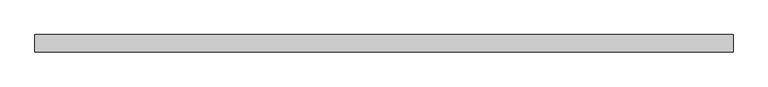
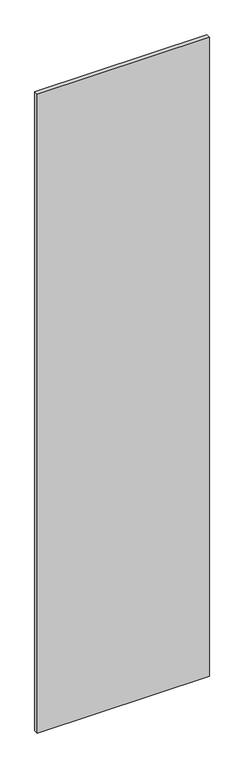
"""IFC4 building model written with IfcOpenShell, lengths in millimetres: plate geometry, 系统嵌板 : 玻璃."""

import ifcopenshell
import ifcopenshell.guid

model = None  # the IFC model being written
_history = None  # IfcOwnerHistory: only IFC2X3 demands one
_inside = {}  # id of a spatial element -> (the spatial element, [elements in it])
_under = {}  # id of a project, library or spatial element -> (it, [spatial elements below it])
_declared = {}  # id of a project -> (the project, [libraries it declares])
_typed = {}  # id of a type object -> (the type object, [elements of that type])
_made_of = {}  # id of a material, layer set ... -> (it, [elements and type objects made of it])


def new_model(schema):
    """Start an empty IFC model of exactly this schema.

    Asked for "IFC4X3", IfcOpenShell would pick the latest addendum, in which some entities
    have other attributes; the version numbers below select the first issue.
    IFC2X3 requires an IfcOwnerHistory on every rooted entity: one is made here for all.
    """
    global model, _history
    if schema == "IFC4X3":
        model = ifcopenshell.file(schema_version=(4, 3, 0, 0))
    else:
        model = ifcopenshell.file(schema=schema)
    _inside.clear()
    _under.clear()
    _declared.clear()
    _typed.clear()
    _made_of.clear()
    _history = None
    if model.schema == "IFC2X3":
        org = make("IfcOrganization", Name="unknown")
        user = make(
            "IfcPersonAndOrganization",
            ThePerson=make("IfcPerson", FamilyName="unknown"),
            TheOrganization=org,
        )
        app = make(
            "IfcApplication",
            ApplicationDeveloper=org,
            Version="unknown",
            ApplicationFullName="unknown",
            ApplicationIdentifier="unknown",
        )
        _history = make(
            "IfcOwnerHistory",
            OwningUser=user,
            OwningApplication=app,
            ChangeAction="ADDED",
            CreationDate=0,
        )
    return model


def make(cls, **values):
    """One entity of the class cls with the attributes given. An attribute that is None is left unset."""
    return model.create_entity(
        cls, **{name: value for name, value in values.items() if value is not None}
    )


def rooted(cls, **values):
    """An entity with a GlobalId (a new one), such as an element, a storey or a relation."""
    return make(cls, GlobalId=ifcopenshell.guid.new(), OwnerHistory=_history, **values)


def si_unit(unit_type, name, prefix=None):
    """IfcSIUnit, for example si_unit("LENGTHUNIT", "METRE", prefix="MILLI")."""
    return make("IfcSIUnit", UnitType=unit_type, Prefix=prefix, Name=name)


def assignment(units):
    """IfcUnitAssignment: the units of a project."""
    return None if units is None else make("IfcUnitAssignment", Units=units)


def point(xyz):
    """IfcCartesianPoint."""
    return None if xyz is None else make("IfcCartesianPoint", Coordinates=xyz)


def direction(xyz):
    """IfcDirection."""
    return None if xyz is None else make("IfcDirection", DirectionRatios=xyz)


def frame(location, z_axis=None, x_axis=None):
    """IfcAxis2Placement3D, a coordinate frame: its origin and axes. An axis left out is left unset."""
    return make(
        "IfcAxis2Placement3D",
        Location=point(location),
        Axis=direction(z_axis),
        RefDirection=direction(x_axis),
    )


def origin():
    """The frame at (0, 0, 0) with its axes left unset."""
    return frame((0.0, 0.0, 0.0))


def origin_with_axes():
    """The frame at (0, 0, 0) with the z axis (0, 0, 1) and the x axis (1, 0, 0) written out."""
    return frame((0.0, 0.0, 0.0), z_axis=(0.0, 0.0, 1.0), x_axis=(1.0, 0.0, 0.0))


def place(relative_to, where):
    """IfcLocalPlacement: puts the frame where relative to a parent placement (None: the world)."""
    return make(
        "IfcLocalPlacement", PlacementRelTo=relative_to, RelativePlacement=where
    )


def context(
    kind, dimensions, precision=None, world=None, true_north=None, identifier=None
):
    """IfcGeometricRepresentationContext, for example the 3D "Model" context."""
    return make(
        "IfcGeometricRepresentationContext",
        ContextIdentifier=identifier,
        ContextType=kind,
        CoordinateSpaceDimension=dimensions,
        Precision=precision,
        WorldCoordinateSystem=world,
        TrueNorth=true_north,
    )


def project(units=None, contexts=None):
    """IfcProject with its units and contexts."""
    return rooted(
        "IfcProject",
        Name="project",
        RepresentationContexts=contexts,
        UnitsInContext=assignment(units),
    )


def spatial(cls, under=None, at=None, **own):
    """A site, building, storey or space (cls), placed at a placement, below another one or the project."""
    s = rooted(cls, ObjectPlacement=at, **own)
    if under is not None:
        _under.setdefault(under.id(), (under, []))[1].append(s)
    return s


def polyline(points):
    """IfcPolyline through the points."""
    return make("IfcPolyline", Points=[point(p) for p in points])


def outline(outer, holes=None, kind="AREA"):
    """IfcArbitraryClosedProfileDef: a profile drawn as a closed curve; with holes, ...WithVoids."""
    if holes is None:
        return make("IfcArbitraryClosedProfileDef", ProfileType=kind, OuterCurve=outer)
    return make(
        "IfcArbitraryProfileDefWithVoids",
        ProfileType=kind,
        OuterCurve=outer,
        InnerCurves=holes,
    )


def extrude(swept, where, along, depth):
    """IfcExtrudedAreaSolid: the profile swept, set in the frame where, extruded along a direction by depth."""
    return make(
        "IfcExtrudedAreaSolid",
        SweptArea=swept,
        Position=where,
        ExtrudedDirection=direction(along),
        Depth=depth,
    )


def shape(context_of_items, identifier, shape_type, items):
    """IfcShapeRepresentation: the items that make up one representation, for example the "Body"."""
    return make(
        "IfcShapeRepresentation",
        ContextOfItems=context_of_items,
        RepresentationIdentifier=identifier,
        RepresentationType=shape_type,
        Items=items,
    )


def source(mapping_origin, context_of_items, identifier, shape_type, items):
    """IfcRepresentationMap: a shape defined once, which mapped items show again and again."""
    return make(
        "IfcRepresentationMap",
        MappingOrigin=mapping_origin,
        MappedRepresentation=shape(context_of_items, identifier, shape_type, items),
    )


def transform(
    local_origin,
    x_axis=None,
    y_axis=None,
    z_axis=None,
    scale=None,
    scale2=None,
    scale3=None,
    uniform=True,
):
    """IfcCartesianTransformationOperator3D, or its non-uniform kind. x_axis, y_axis, z_axis: its Axis1, 2, 3."""
    if uniform:
        return make(
            "IfcCartesianTransformationOperator3D",
            Axis1=direction(x_axis),
            Axis2=direction(y_axis),
            LocalOrigin=point(local_origin),
            Scale=scale,
            Axis3=direction(z_axis),
        )
    return make(
        "IfcCartesianTransformationOperator3DnonUniform",
        Axis1=direction(x_axis),
        Axis2=direction(y_axis),
        LocalOrigin=point(local_origin),
        Scale=scale,
        Axis3=direction(z_axis),
        Scale2=scale2,
        Scale3=scale3,
    )


def mapped(mapping_source, mapping_target):
    """IfcMappedItem: shows the shape of a source again, moved by a transform."""
    return make(
        "IfcMappedItem", MappingSource=mapping_source, MappingTarget=mapping_target
    )


def made_of(thing, what):
    """Note that an element or type object is made of a material, layer set ...; save() writes the relation."""
    if what is not None:
        _made_of.setdefault(what.id(), (what, []))[1].append(thing)
    return thing


def element(
    cls,
    number,
    at=None,
    inside=None,
    cuts=None,
    type_object=None,
    material=None,
    context=None,
    identifier="Body",
    shape_type=None,
    held_by="IfcProductDefinitionShape",
    body=None,
    shapes=None,
    **own,
):
    """One element of the class cls, such as IfcWall. Its Tag is "e" and its number.

    at: its placement. inside: the storey or other place that contains it. cuts: it is an
    opening in that element (IfcRelVoidsElement). A single representation is given by context,
    identifier, shape_type and body (its items); several are given by shapes. held_by: the class
    of the entity that holds the representations. save() writes the other relations.
    """
    e = rooted(cls, Tag="e%d" % number, ObjectPlacement=at, **own)
    if body is not None:
        shapes = [shape(context, identifier, shape_type, body)]
    if shapes is not None:
        e.Representation = make(held_by, Representations=shapes)
    if inside is not None:
        _inside.setdefault(inside.id(), (inside, []))[1].append(e)
    if cuts is not None:
        rooted(
            "IfcRelVoidsElement", RelatingBuildingElement=cuts, RelatedOpeningElement=e
        )
    if type_object is not None:
        _typed.setdefault(type_object.id(), (type_object, []))[1].append(e)
    return made_of(e, material)


def aggregate(whole, parts):
    """IfcRelAggregates: a whole, such as a stair, and the parts it consists of."""
    return rooted("IfcRelAggregates", RelatingObject=whole, RelatedObjects=parts)


def save(model, path):
    """Write the relations noted so far, then the file.

    IfcRelAggregates (storeys below a building ...), IfcRelContainedInSpatialStructure (elements
    in a storey), IfcRelDefinesByType, IfcRelAssociatesMaterial and IfcRelDeclares: one each for
    every whole, place, type object, material and project.
    """
    for whole, parts in _under.values():
        aggregate(whole, parts)
    for where, things in _inside.values():
        rooted(
            "IfcRelContainedInSpatialStructure",
            RelatedElements=things,
            RelatingStructure=where,
        )
    for kind, things in _typed.values():
        rooted("IfcRelDefinesByType", RelatedObjects=things, RelatingType=kind)
    for what, things in _made_of.values():
        rooted("IfcRelAssociatesMaterial", RelatedObjects=things, RelatingMaterial=what)
    for by, libraries in _declared.values():
        rooted("IfcRelDeclares", RelatingContext=by, RelatedDefinitions=libraries)
    model.write(path)


def plate_1e3715b7(model_context):
    return source(origin(), model_context, "Body", "SweptSolid", [
        extrude(outline(polyline([(510.0, -12.5), (-510.0, -12.5), (-510.0, 12.5), (510.0, 12.5), (510.0, -12.5)])), origin_with_axes(), (0.0, 0.0, 1.0), 4000.0),
    ])


if __name__ == "__main__":
    model = new_model("IFC4")
    model_context = context("Model", 3, world=origin())
    ifc_project = project(units=[si_unit("LENGTHUNIT", "METRE", prefix="MILLI")], contexts=[model_context])
    site = spatial("IfcSite", under=ifc_project)
    building = spatial("IfcBuilding", under=site)
    placement = place(None, origin())
    plate_shape = plate_1e3715b7(model_context)
    element("IfcPlate", 1, ObjectType="系统嵌板 : 玻璃", at=placement, inside=building, context=model_context, shape_type="MappedRepresentation", body=[
        mapped(plate_shape, transform((0.0, 0.0, 0.0), x_axis=(1.0, 0.0, 0.0), y_axis=(0.0, 1.0, 0.0), z_axis=(0.0, 0.0, 1.0))),
    ])
    save(model, "model.ifc")

# Revit data of these elements
# Type "系统嵌板 : 玻璃"
#   Construction Type Id = "GSP4R"
#   Analytic Construction = "1/8 英寸 Pilkington 单层玻璃"
#   Visual Light Transmittance = 0.9
#   Solar Heat Gain Coefficient = 0.86
#   Heat Transfer Coefficient (U) = 6.7069 W/(m²·K)
# Element 1 (IfcPlate, "系统嵌板 : 玻璃")
#   Materials on its faces: "玻璃"
# Materials
#   "玻璃": class "玻璃", colour RGB 0 128 192, transparency 0.9, Description = "钠钙玻璃", Cost = 0
